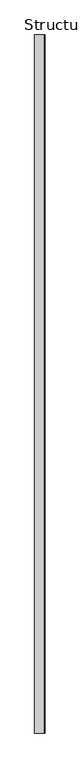
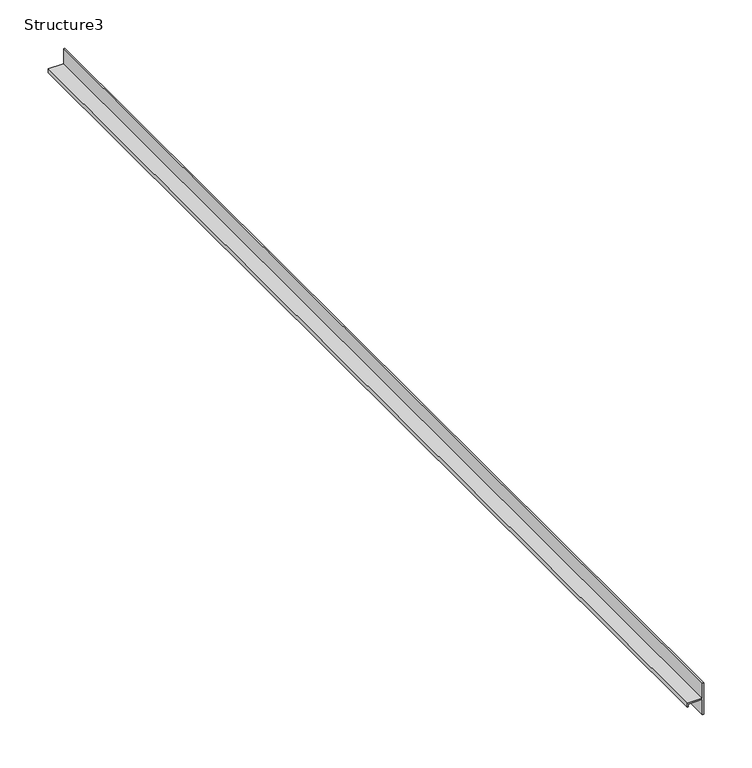
"""IFC4 building model written with IfcOpenShell, lengths in millimetres: proxy geometry, Structure3 : Structure668217158."""

from ifc_helpers import new_model, si_unit, frame, origin, place, context, project, spatial, polyline, outline, extrude, source, transform, mapped, element, save


def structure3_3761bdce(model_context):
    return source(origin(), model_context, "Body", "SweptSolid", [
        extrude(outline(polyline([(40092.376, 10286.0440827), (40073.326, 10286.0440827), (40073.326, 10287.3140827), (40112.696, 10287.3140827), (40112.696, 10286.0440827), (40093.646, 10286.0440827), (40093.646, 10267.8101348), (40088.8962, 10267.8101348), (40088.8962, 10269.0801348), (40092.376, 10269.0801348), (40092.376, 10286.0440827)])), frame((0.0, 559.3171815, 0.0), z_axis=(0.0, 1.0, 0.0), x_axis=(0.0, 0.0, 1.0)), (0.0, 0.0, 1.0), 1319.9959487),
    ])


if __name__ == "__main__":
    model = new_model("IFC4")
    model_context = context("Model", 3, world=origin())
    ifc_project = project(units=[si_unit("LENGTHUNIT", "METRE", prefix="MILLI")], contexts=[model_context])
    site = spatial("IfcSite", under=ifc_project)
    building = spatial("IfcBuilding", under=site)
    placement = place(None, origin())
    structure3_shape = structure3_3761bdce(model_context)
    element("IfcBuildingElementProxy", 1, Name="Structure3 : Structure668217158", ObjectType="Structure3 : Structure668217158", at=placement, inside=building, context=model_context, shape_type="MappedRepresentation", body=[
        mapped(structure3_shape, transform((0.0, 0.0, 0.0), x_axis=(1.0, 0.0, 0.0), y_axis=(0.0, 1.0, 0.0), z_axis=(0.0, 0.0, 1.0))),
    ])
    save(model, "model.ifc")

# Revit data of these elements
# Type "Structure3 : Structure668217158"
#   NameOverride = "Structure668217158"
# Element 1 (IfcBuildingElementProxy, "Structure3 : Structure668217158")
#   Materials on its faces: "DRYWALL REVEAL BEAD"
# Materials
#   "DRYWALL REVEAL BEAD": class "Unassigned", colour RGB 255 241 0, transparency 0, Cost = 0
